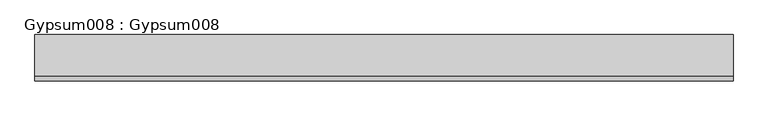
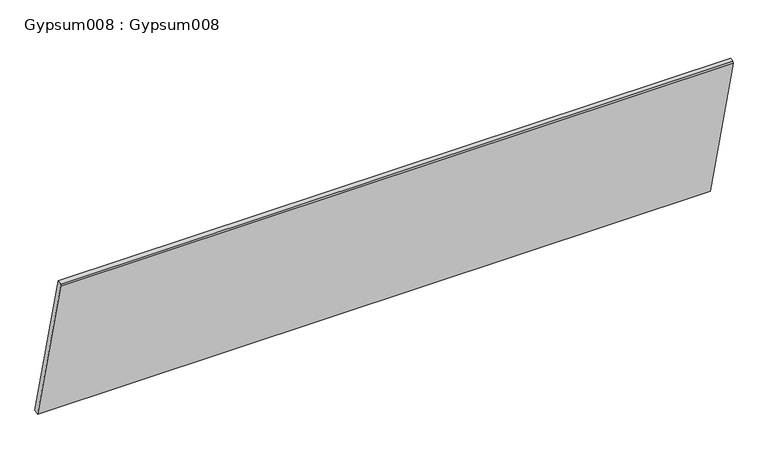
"""IFC4 building model written with IfcOpenShell, lengths in millimetres: proxy geometry, Gypsum008 : Gypsum008."""

import ifcopenshell
import ifcopenshell.guid

model = None  # the IFC model being written
_history = None  # IfcOwnerHistory: only IFC2X3 demands one
_inside = {}  # id of a spatial element -> (the spatial element, [elements in it])
_under = {}  # id of a project, library or spatial element -> (it, [spatial elements below it])
_declared = {}  # id of a project -> (the project, [libraries it declares])
_typed = {}  # id of a type object -> (the type object, [elements of that type])
_made_of = {}  # id of a material, layer set ... -> (it, [elements and type objects made of it])


def new_model(schema):
    """Start an empty IFC model of exactly this schema.

    Asked for "IFC4X3", IfcOpenShell would pick the latest addendum, in which some entities
    have other attributes; the version numbers below select the first issue.
    IFC2X3 requires an IfcOwnerHistory on every rooted entity: one is made here for all.
    """
    global model, _history
    if schema == "IFC4X3":
        model = ifcopenshell.file(schema_version=(4, 3, 0, 0))
    else:
        model = ifcopenshell.file(schema=schema)
    _inside.clear()
    _under.clear()
    _declared.clear()
    _typed.clear()
    _made_of.clear()
    _history = None
    if model.schema == "IFC2X3":
        org = make("IfcOrganization", Name="unknown")
        user = make(
            "IfcPersonAndOrganization",
            ThePerson=make("IfcPerson", FamilyName="unknown"),
            TheOrganization=org,
        )
        app = make(
            "IfcApplication",
            ApplicationDeveloper=org,
            Version="unknown",
            ApplicationFullName="unknown",
            ApplicationIdentifier="unknown",
        )
        _history = make(
            "IfcOwnerHistory",
            OwningUser=user,
            OwningApplication=app,
            ChangeAction="ADDED",
            CreationDate=0,
        )
    return model


def make(cls, **values):
    """One entity of the class cls with the attributes given. An attribute that is None is left unset."""
    return model.create_entity(
        cls, **{name: value for name, value in values.items() if value is not None}
    )


def rooted(cls, **values):
    """An entity with a GlobalId (a new one), such as an element, a storey or a relation."""
    return make(cls, GlobalId=ifcopenshell.guid.new(), OwnerHistory=_history, **values)


def si_unit(unit_type, name, prefix=None):
    """IfcSIUnit, for example si_unit("LENGTHUNIT", "METRE", prefix="MILLI")."""
    return make("IfcSIUnit", UnitType=unit_type, Prefix=prefix, Name=name)


def assignment(units):
    """IfcUnitAssignment: the units of a project."""
    return None if units is None else make("IfcUnitAssignment", Units=units)


def point(xyz):
    """IfcCartesianPoint."""
    return None if xyz is None else make("IfcCartesianPoint", Coordinates=xyz)


def direction(xyz):
    """IfcDirection."""
    return None if xyz is None else make("IfcDirection", DirectionRatios=xyz)


def frame(location, z_axis=None, x_axis=None):
    """IfcAxis2Placement3D, a coordinate frame: its origin and axes. An axis left out is left unset."""
    return make(
        "IfcAxis2Placement3D",
        Location=point(location),
        Axis=direction(z_axis),
        RefDirection=direction(x_axis),
    )


def origin():
    """The frame at (0, 0, 0) with its axes left unset."""
    return frame((0.0, 0.0, 0.0))


def place(relative_to, where):
    """IfcLocalPlacement: puts the frame where relative to a parent placement (None: the world)."""
    return make(
        "IfcLocalPlacement", PlacementRelTo=relative_to, RelativePlacement=where
    )


def context(
    kind, dimensions, precision=None, world=None, true_north=None, identifier=None
):
    """IfcGeometricRepresentationContext, for example the 3D "Model" context."""
    return make(
        "IfcGeometricRepresentationContext",
        ContextIdentifier=identifier,
        ContextType=kind,
        CoordinateSpaceDimension=dimensions,
        Precision=precision,
        WorldCoordinateSystem=world,
        TrueNorth=true_north,
    )


def project(units=None, contexts=None):
    """IfcProject with its units and contexts."""
    return rooted(
        "IfcProject",
        Name="project",
        RepresentationContexts=contexts,
        UnitsInContext=assignment(units),
    )


def spatial(cls, under=None, at=None, **own):
    """A site, building, storey or space (cls), placed at a placement, below another one or the project."""
    s = rooted(cls, ObjectPlacement=at, **own)
    if under is not None:
        _under.setdefault(under.id(), (under, []))[1].append(s)
    return s


def polyline(points):
    """IfcPolyline through the points."""
    return make("IfcPolyline", Points=[point(p) for p in points])


def outline(outer, holes=None, kind="AREA"):
    """IfcArbitraryClosedProfileDef: a profile drawn as a closed curve; with holes, ...WithVoids."""
    if holes is None:
        return make("IfcArbitraryClosedProfileDef", ProfileType=kind, OuterCurve=outer)
    return make(
        "IfcArbitraryProfileDefWithVoids",
        ProfileType=kind,
        OuterCurve=outer,
        InnerCurves=holes,
    )


def extrude(swept, where, along, depth):
    """IfcExtrudedAreaSolid: the profile swept, set in the frame where, extruded along a direction by depth."""
    return make(
        "IfcExtrudedAreaSolid",
        SweptArea=swept,
        Position=where,
        ExtrudedDirection=direction(along),
        Depth=depth,
    )


def shape(context_of_items, identifier, shape_type, items):
    """IfcShapeRepresentation: the items that make up one representation, for example the "Body"."""
    return make(
        "IfcShapeRepresentation",
        ContextOfItems=context_of_items,
        RepresentationIdentifier=identifier,
        RepresentationType=shape_type,
        Items=items,
    )


def source(mapping_origin, context_of_items, identifier, shape_type, items):
    """IfcRepresentationMap: a shape defined once, which mapped items show again and again."""
    return make(
        "IfcRepresentationMap",
        MappingOrigin=mapping_origin,
        MappedRepresentation=shape(context_of_items, identifier, shape_type, items),
    )


def transform(
    local_origin,
    x_axis=None,
    y_axis=None,
    z_axis=None,
    scale=None,
    scale2=None,
    scale3=None,
    uniform=True,
):
    """IfcCartesianTransformationOperator3D, or its non-uniform kind. x_axis, y_axis, z_axis: its Axis1, 2, 3."""
    if uniform:
        return make(
            "IfcCartesianTransformationOperator3D",
            Axis1=direction(x_axis),
            Axis2=direction(y_axis),
            LocalOrigin=point(local_origin),
            Scale=scale,
            Axis3=direction(z_axis),
        )
    return make(
        "IfcCartesianTransformationOperator3DnonUniform",
        Axis1=direction(x_axis),
        Axis2=direction(y_axis),
        LocalOrigin=point(local_origin),
        Scale=scale,
        Axis3=direction(z_axis),
        Scale2=scale2,
        Scale3=scale3,
    )


def mapped(mapping_source, mapping_target):
    """IfcMappedItem: shows the shape of a source again, moved by a transform."""
    return make(
        "IfcMappedItem", MappingSource=mapping_source, MappingTarget=mapping_target
    )


def made_of(thing, what):
    """Note that an element or type object is made of a material, layer set ...; save() writes the relation."""
    if what is not None:
        _made_of.setdefault(what.id(), (what, []))[1].append(thing)
    return thing


def element(
    cls,
    number,
    at=None,
    inside=None,
    cuts=None,
    type_object=None,
    material=None,
    context=None,
    identifier="Body",
    shape_type=None,
    held_by="IfcProductDefinitionShape",
    body=None,
    shapes=None,
    **own,
):
    """One element of the class cls, such as IfcWall. Its Tag is "e" and its number.

    at: its placement. inside: the storey or other place that contains it. cuts: it is an
    opening in that element (IfcRelVoidsElement). A single representation is given by context,
    identifier, shape_type and body (its items); several are given by shapes. held_by: the class
    of the entity that holds the representations. save() writes the other relations.
    """
    e = rooted(cls, Tag="e%d" % number, ObjectPlacement=at, **own)
    if body is not None:
        shapes = [shape(context, identifier, shape_type, body)]
    if shapes is not None:
        e.Representation = make(held_by, Representations=shapes)
    if inside is not None:
        _inside.setdefault(inside.id(), (inside, []))[1].append(e)
    if cuts is not None:
        rooted(
            "IfcRelVoidsElement", RelatingBuildingElement=cuts, RelatedOpeningElement=e
        )
    if type_object is not None:
        _typed.setdefault(type_object.id(), (type_object, []))[1].append(e)
    return made_of(e, material)


def aggregate(whole, parts):
    """IfcRelAggregates: a whole, such as a stair, and the parts it consists of."""
    return rooted("IfcRelAggregates", RelatingObject=whole, RelatedObjects=parts)


def save(model, path):
    """Write the relations noted so far, then the file.

    IfcRelAggregates (storeys below a building ...), IfcRelContainedInSpatialStructure (elements
    in a storey), IfcRelDefinesByType, IfcRelAssociatesMaterial and IfcRelDeclares: one each for
    every whole, place, type object, material and project.
    """
    for whole, parts in _under.values():
        aggregate(whole, parts)
    for where, things in _inside.values():
        rooted(
            "IfcRelContainedInSpatialStructure",
            RelatedElements=things,
            RelatingStructure=where,
        )
    for kind, things in _typed.values():
        rooted("IfcRelDefinesByType", RelatedObjects=things, RelatingType=kind)
    for what, things in _made_of.values():
        rooted("IfcRelAssociatesMaterial", RelatedObjects=things, RelatingMaterial=what)
    for by, libraries in _declared.values():
        rooted("IfcRelDeclares", RelatingContext=by, RelatedDefinitions=libraries)
    model.write(path)


def gypsum008_gypsum008_d0d3208e(model_context):
    return source(origin(), model_context, "Body", "SweptSolid", [
        extrude(outline(polyline([(9752.047493, 43222.0071182), (9737.9368073, 43218.4770293), (9619.3816911, 43692.3727377), (9619.9854477, 43698.7661533), (9632.0226951, 43701.7775274), (9752.047493, 43222.0071182)])), frame((3694.2883192, 0.0, 0.0), z_axis=(1.0, 0.0, 0.0), x_axis=(0.0, 1.0, 0.0)), (0.0, 0.0, 1.0), 2000.0),
    ])


if __name__ == "__main__":
    model = new_model("IFC4")
    model_context = context("Model", 3, world=origin())
    ifc_project = project(units=[si_unit("LENGTHUNIT", "METRE", prefix="MILLI")], contexts=[model_context])
    site = spatial("IfcSite", under=ifc_project)
    building = spatial("IfcBuilding", under=site)
    placement = place(None, origin())
    gypsum008_gypsum008_shape = gypsum008_gypsum008_d0d3208e(model_context)
    element("IfcBuildingElementProxy", 1, Name="Gypsum008 : Gypsum008", ObjectType="Gypsum008 : Gypsum008", at=placement, inside=building, context=model_context, shape_type="MappedRepresentation", body=[
        mapped(gypsum008_gypsum008_shape, transform((0.0, 0.0, 0.0), x_axis=(1.0, 0.0, 0.0), y_axis=(0.0, 1.0, 0.0), z_axis=(0.0, 0.0, 1.0))),
    ])
    save(model, "model.ifc")

# Revit data of these elements
# Type "Gypsum008 : Gypsum008"
#   NameOverride = "Gypsum008"
# Element 1 (IfcBuildingElementProxy, "Gypsum008 : Gypsum008")
#   Materials on its faces: "5/8\" GYPSUM BOARD 912"
# Materials
#   "5/8\" GYPSUM BOARD 912": class "Unassigned", colour RGB 206 255 255, transparency 0
